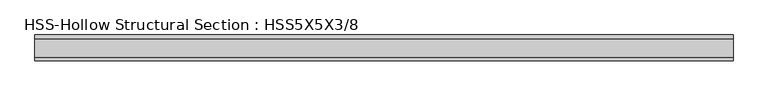
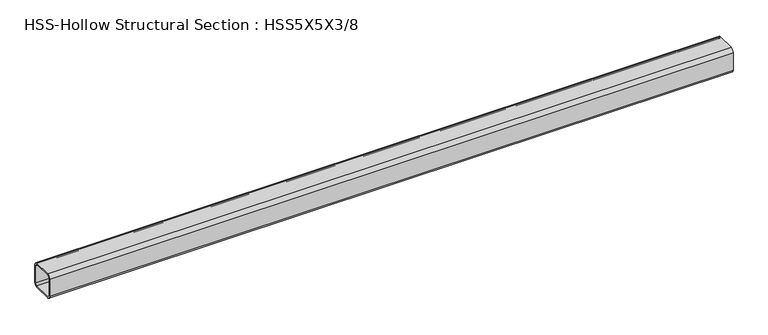
"""IFC4 building model written with IfcOpenShell, lengths in millimetres: member geometry, HSS-Hollow Structural Section : HSS5X5X3/8."""

import ifcopenshell
import ifcopenshell.guid

model = None  # the IFC model being written
_history = None  # IfcOwnerHistory: only IFC2X3 demands one
_inside = {}  # id of a spatial element -> (the spatial element, [elements in it])
_under = {}  # id of a project, library or spatial element -> (it, [spatial elements below it])
_declared = {}  # id of a project -> (the project, [libraries it declares])
_typed = {}  # id of a type object -> (the type object, [elements of that type])
_made_of = {}  # id of a material, layer set ... -> (it, [elements and type objects made of it])


def new_model(schema):
    """Start an empty IFC model of exactly this schema.

    Asked for "IFC4X3", IfcOpenShell would pick the latest addendum, in which some entities
    have other attributes; the version numbers below select the first issue.
    IFC2X3 requires an IfcOwnerHistory on every rooted entity: one is made here for all.
    """
    global model, _history
    if schema == "IFC4X3":
        model = ifcopenshell.file(schema_version=(4, 3, 0, 0))
    else:
        model = ifcopenshell.file(schema=schema)
    _inside.clear()
    _under.clear()
    _declared.clear()
    _typed.clear()
    _made_of.clear()
    _history = None
    if model.schema == "IFC2X3":
        org = make("IfcOrganization", Name="unknown")
        user = make(
            "IfcPersonAndOrganization",
            ThePerson=make("IfcPerson", FamilyName="unknown"),
            TheOrganization=org,
        )
        app = make(
            "IfcApplication",
            ApplicationDeveloper=org,
            Version="unknown",
            ApplicationFullName="unknown",
            ApplicationIdentifier="unknown",
        )
        _history = make(
            "IfcOwnerHistory",
            OwningUser=user,
            OwningApplication=app,
            ChangeAction="ADDED",
            CreationDate=0,
        )
    return model


def make(cls, **values):
    """One entity of the class cls with the attributes given. An attribute that is None is left unset."""
    return model.create_entity(
        cls, **{name: value for name, value in values.items() if value is not None}
    )


def rooted(cls, **values):
    """An entity with a GlobalId (a new one), such as an element, a storey or a relation."""
    return make(cls, GlobalId=ifcopenshell.guid.new(), OwnerHistory=_history, **values)


def si_unit(unit_type, name, prefix=None):
    """IfcSIUnit, for example si_unit("LENGTHUNIT", "METRE", prefix="MILLI")."""
    return make("IfcSIUnit", UnitType=unit_type, Prefix=prefix, Name=name)


def assignment(units):
    """IfcUnitAssignment: the units of a project."""
    return None if units is None else make("IfcUnitAssignment", Units=units)


def point(xyz):
    """IfcCartesianPoint."""
    return None if xyz is None else make("IfcCartesianPoint", Coordinates=xyz)


def direction(xyz):
    """IfcDirection."""
    return None if xyz is None else make("IfcDirection", DirectionRatios=xyz)


def frame(location, z_axis=None, x_axis=None):
    """IfcAxis2Placement3D, a coordinate frame: its origin and axes. An axis left out is left unset."""
    return make(
        "IfcAxis2Placement3D",
        Location=point(location),
        Axis=direction(z_axis),
        RefDirection=direction(x_axis),
    )


def frame_2d(location, x_axis=None):
    """IfcAxis2Placement2D, a coordinate frame in the plane: its origin and x axis."""
    return make(
        "IfcAxis2Placement2D", Location=point(location), RefDirection=direction(x_axis)
    )


def origin():
    """The frame at (0, 0, 0) with its axes left unset."""
    return frame((0.0, 0.0, 0.0))


def place(relative_to, where):
    """IfcLocalPlacement: puts the frame where relative to a parent placement (None: the world)."""
    return make(
        "IfcLocalPlacement", PlacementRelTo=relative_to, RelativePlacement=where
    )


def context(
    kind, dimensions, precision=None, world=None, true_north=None, identifier=None
):
    """IfcGeometricRepresentationContext, for example the 3D "Model" context."""
    return make(
        "IfcGeometricRepresentationContext",
        ContextIdentifier=identifier,
        ContextType=kind,
        CoordinateSpaceDimension=dimensions,
        Precision=precision,
        WorldCoordinateSystem=world,
        TrueNorth=true_north,
    )


def project(units=None, contexts=None):
    """IfcProject with its units and contexts."""
    return rooted(
        "IfcProject",
        Name="project",
        RepresentationContexts=contexts,
        UnitsInContext=assignment(units),
    )


def spatial(cls, under=None, at=None, **own):
    """A site, building, storey or space (cls), placed at a placement, below another one or the project."""
    s = rooted(cls, ObjectPlacement=at, **own)
    if under is not None:
        _under.setdefault(under.id(), (under, []))[1].append(s)
    return s


def polyline(points):
    """IfcPolyline through the points."""
    return make("IfcPolyline", Points=[point(p) for p in points])


def circle_curve(where, radius):
    """IfcCircle in the frame where."""
    return make("IfcCircle", Position=where, Radius=radius)


def trimmed(basis, trim1, trim2, sense, master):
    """IfcTrimmedCurve: the piece of a basis curve between two trims."""
    return make(
        "IfcTrimmedCurve",
        BasisCurve=basis,
        Trim1=trim1,
        Trim2=trim2,
        SenseAgreement=sense,
        MasterRepresentation=master,
    )


def segment(curve, same_sense, transition):
    """IfcCompositeCurveSegment."""
    return make(
        "IfcCompositeCurveSegment",
        Transition=transition,
        SameSense=same_sense,
        ParentCurve=curve,
    )


def composite_curve(segments, self_intersect=None):
    """IfcCompositeCurve: segments joined end to end."""
    return make("IfcCompositeCurve", Segments=segments, SelfIntersect=self_intersect)


def outline(outer, holes=None, kind="AREA"):
    """IfcArbitraryClosedProfileDef: a profile drawn as a closed curve; with holes, ...WithVoids."""
    if holes is None:
        return make("IfcArbitraryClosedProfileDef", ProfileType=kind, OuterCurve=outer)
    return make(
        "IfcArbitraryProfileDefWithVoids",
        ProfileType=kind,
        OuterCurve=outer,
        InnerCurves=holes,
    )


def extrude(swept, where, along, depth):
    """IfcExtrudedAreaSolid: the profile swept, set in the frame where, extruded along a direction by depth."""
    return make(
        "IfcExtrudedAreaSolid",
        SweptArea=swept,
        Position=where,
        ExtrudedDirection=direction(along),
        Depth=depth,
    )


def shape(context_of_items, identifier, shape_type, items):
    """IfcShapeRepresentation: the items that make up one representation, for example the "Body"."""
    return make(
        "IfcShapeRepresentation",
        ContextOfItems=context_of_items,
        RepresentationIdentifier=identifier,
        RepresentationType=shape_type,
        Items=items,
    )


def source(mapping_origin, context_of_items, identifier, shape_type, items):
    """IfcRepresentationMap: a shape defined once, which mapped items show again and again."""
    return make(
        "IfcRepresentationMap",
        MappingOrigin=mapping_origin,
        MappedRepresentation=shape(context_of_items, identifier, shape_type, items),
    )


def transform(
    local_origin,
    x_axis=None,
    y_axis=None,
    z_axis=None,
    scale=None,
    scale2=None,
    scale3=None,
    uniform=True,
):
    """IfcCartesianTransformationOperator3D, or its non-uniform kind. x_axis, y_axis, z_axis: its Axis1, 2, 3."""
    if uniform:
        return make(
            "IfcCartesianTransformationOperator3D",
            Axis1=direction(x_axis),
            Axis2=direction(y_axis),
            LocalOrigin=point(local_origin),
            Scale=scale,
            Axis3=direction(z_axis),
        )
    return make(
        "IfcCartesianTransformationOperator3DnonUniform",
        Axis1=direction(x_axis),
        Axis2=direction(y_axis),
        LocalOrigin=point(local_origin),
        Scale=scale,
        Axis3=direction(z_axis),
        Scale2=scale2,
        Scale3=scale3,
    )


def mapped(mapping_source, mapping_target):
    """IfcMappedItem: shows the shape of a source again, moved by a transform."""
    return make(
        "IfcMappedItem", MappingSource=mapping_source, MappingTarget=mapping_target
    )


def made_of(thing, what):
    """Note that an element or type object is made of a material, layer set ...; save() writes the relation."""
    if what is not None:
        _made_of.setdefault(what.id(), (what, []))[1].append(thing)
    return thing


def element(
    cls,
    number,
    at=None,
    inside=None,
    cuts=None,
    type_object=None,
    material=None,
    context=None,
    identifier="Body",
    shape_type=None,
    held_by="IfcProductDefinitionShape",
    body=None,
    shapes=None,
    **own,
):
    """One element of the class cls, such as IfcWall. Its Tag is "e" and its number.

    at: its placement. inside: the storey or other place that contains it. cuts: it is an
    opening in that element (IfcRelVoidsElement). A single representation is given by context,
    identifier, shape_type and body (its items); several are given by shapes. held_by: the class
    of the entity that holds the representations. save() writes the other relations.
    """
    e = rooted(cls, Tag="e%d" % number, ObjectPlacement=at, **own)
    if body is not None:
        shapes = [shape(context, identifier, shape_type, body)]
    if shapes is not None:
        e.Representation = make(held_by, Representations=shapes)
    if inside is not None:
        _inside.setdefault(inside.id(), (inside, []))[1].append(e)
    if cuts is not None:
        rooted(
            "IfcRelVoidsElement", RelatingBuildingElement=cuts, RelatedOpeningElement=e
        )
    if type_object is not None:
        _typed.setdefault(type_object.id(), (type_object, []))[1].append(e)
    return made_of(e, material)


def aggregate(whole, parts):
    """IfcRelAggregates: a whole, such as a stair, and the parts it consists of."""
    return rooted("IfcRelAggregates", RelatingObject=whole, RelatedObjects=parts)


def save(model, path):
    """Write the relations noted so far, then the file.

    IfcRelAggregates (storeys below a building ...), IfcRelContainedInSpatialStructure (elements
    in a storey), IfcRelDefinesByType, IfcRelAssociatesMaterial and IfcRelDeclares: one each for
    every whole, place, type object, material and project.
    """
    for whole, parts in _under.values():
        aggregate(whole, parts)
    for where, things in _inside.values():
        rooted(
            "IfcRelContainedInSpatialStructure",
            RelatedElements=things,
            RelatingStructure=where,
        )
    for kind, things in _typed.values():
        rooted("IfcRelDefinesByType", RelatedObjects=things, RelatingType=kind)
    for what, things in _made_of.values():
        rooted("IfcRelAssociatesMaterial", RelatedObjects=things, RelatingMaterial=what)
    for by, libraries in _declared.values():
        rooted("IfcRelDeclares", RelatingContext=by, RelatedDefinitions=libraries)
    model.write(path)


def hss_hollow_structural_section_hss5x5x3_8_c527732f(model_context):
    return source(origin(), model_context, "Body", "SweptSolid", [
        extrude(outline(composite_curve([segment(polyline([(63.5, 45.7708), (63.5, -45.7708)]), True, "CONTINUOUS"), segment(trimmed(circle_curve(frame_2d((45.7708, -45.7708)), 17.7292), [point((63.5, -45.7708))], [point((45.7708, -63.5))], False, "CARTESIAN"), True, "CONTINUOUS"), segment(polyline([(45.7708, -63.5), (-45.7708, -63.5)]), True, "CONTINUOUS"), segment(trimmed(circle_curve(frame_2d((-45.7708, -45.7708)), 17.7292), [point((-45.7708, -63.5))], [point((-63.5, -45.7708))], False, "CARTESIAN"), True, "CONTINUOUS"), segment(polyline([(-63.5, -45.7708), (-63.5, 45.7708)]), True, "CONTINUOUS"), segment(trimmed(circle_curve(frame_2d((-45.7708, 45.7708)), 17.7292), [point((-63.5, 45.7708))], [point((-45.7708, 63.5))], False, "CARTESIAN"), True, "CONTINUOUS"), segment(polyline([(-45.7708, 63.5), (45.7708, 63.5)]), True, "CONTINUOUS"), segment(trimmed(circle_curve(frame_2d((45.7708, 45.7708)), 17.7292), [point((45.7708, 63.5))], [point((63.5, 45.7708))], False, "CARTESIAN"), True, "CONTINUOUS")], self_intersect=False), holes=[composite_curve([segment(trimmed(circle_curve(frame_2d((-45.7708, 45.7708)), 8.8646), [point((-45.7708, 54.6354))], [point((-54.6354, 45.7708))], True, "CARTESIAN"), True, "CONTINUOUS"), segment(polyline([(-54.6354, 45.7708), (-54.6354, -45.7708)]), True, "CONTINUOUS"), segment(trimmed(circle_curve(frame_2d((-45.7708, -45.7708)), 8.8646), [point((-54.6354, -45.7708))], [point((-45.7708, -54.6354))], True, "CARTESIAN"), True, "CONTINUOUS"), segment(polyline([(-45.7708, -54.6354), (45.7708, -54.6354)]), True, "CONTINUOUS"), segment(trimmed(circle_curve(frame_2d((45.7708, -45.7708)), 8.8646), [point((45.7708, -54.6354))], [point((54.6354, -45.7708))], True, "CARTESIAN"), True, "CONTINUOUS"), segment(polyline([(54.6354, -45.7708), (54.6354, 45.7708)]), True, "CONTINUOUS"), segment(trimmed(circle_curve(frame_2d((45.7708, 45.7708)), 8.8646), [point((54.6354, 45.7708))], [point((45.7708, 54.6354))], True, "CARTESIAN"), True, "CONTINUOUS"), segment(polyline([(45.7708, 54.6354), (-45.7708, 54.6354)]), True, "CONTINUOUS")], self_intersect=False)]), frame((-1676.7459948, 0.0, 0.0), z_axis=(1.0, 0.0, 0.0), x_axis=(0.0, 1.0, 0.0)), (0.0, 0.0, 1.0), 3423.5379874),
    ])


if __name__ == "__main__":
    model = new_model("IFC4")
    model_context = context("Model", 3, world=origin())
    ifc_project = project(units=[si_unit("LENGTHUNIT", "METRE", prefix="MILLI")], contexts=[model_context])
    site = spatial("IfcSite", under=ifc_project)
    building = spatial("IfcBuilding", under=site)
    placement = place(None, origin())
    hss_hollow_structural_section_hss5x5x3_8_shape = hss_hollow_structural_section_hss5x5x3_8_c527732f(model_context)
    element("IfcMember", 1, ObjectType="HSS-Hollow Structural Section : HSS5X5X3/8", at=placement, inside=building, context=model_context, shape_type="MappedRepresentation", body=[
        mapped(hss_hollow_structural_section_hss5x5x3_8_shape, transform((0.0, 0.0, 0.0), x_axis=(1.0, 0.0, 0.0), y_axis=(0.0, 1.0, 0.0), z_axis=(0.0, 0.0, 1.0))),
    ])
    save(model, "model.ifc")

# Revit data of these elements
# Type "HSS-Hollow Structural Section : HSS5X5X3/8"
#   Assembly Code = "B10"
#   Shape = "Square"
#   W = 22.3
#   Ht = 0' - 5"
#   Length [instance default] = 5' - 0"
#   b = 0' - 5"
#   kr = 0' - 0.698"
#   t = 0' - 0.349"
#   A = 0.0429167 SF
#   Structural Material [instance default] = Steel ASTM A500, Grade B, Rectangular and Square
# Element 1 (IfcMember, "HSS-Hollow Structural Section : HSS5X5X3/8")
#   Materials on its faces: "Steel ASTM A500, Grade B, Rectangular and Square"
# Materials
#   "Steel ASTM A500, Grade B, Rectangular and Square": class "Metal", colour RGB 199 199 199, transparency 0, Description = "Carbon steel", Cost = 0
